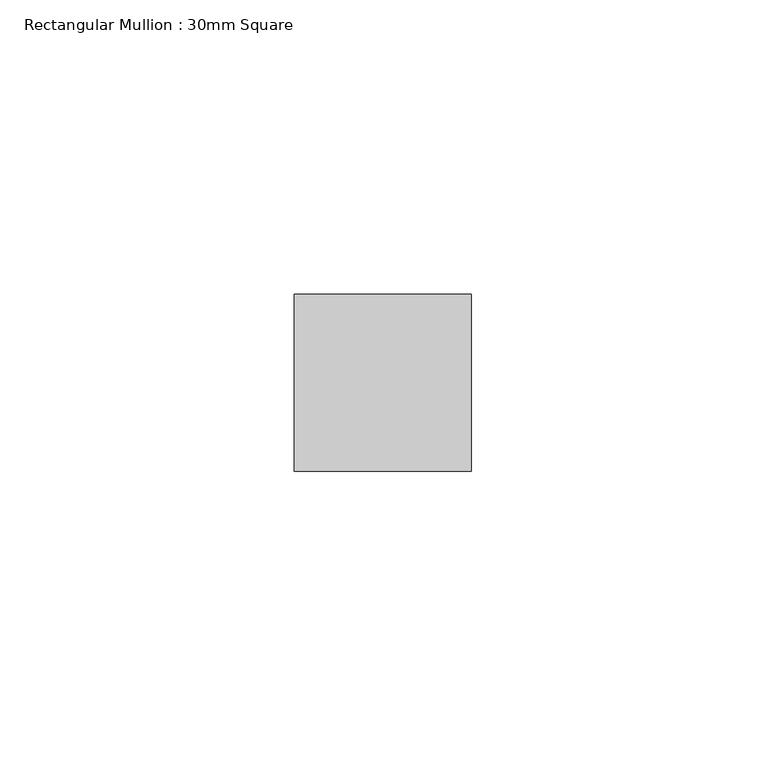
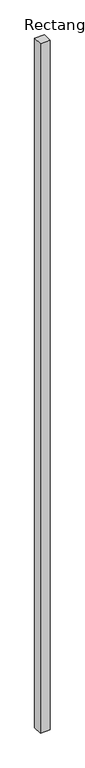
"""IFC4 building model written with IfcOpenShell, lengths in millimetres: member geometry, Rectangular Mullion : 30mm Square."""

from ifc_helpers import new_model, si_unit, frame, origin, place, context, project, spatial, polyline, outline, extrude, source, transform, mapped, element, save


def rectangular_mullion_30mm_square_b3fc8657(model_context):
    return source(origin(), model_context, "Body", "SweptSolid", [
        extrude(outline(polyline([(15.0, 15.0), (15.0, -15.0), (-15.0, -15.0), (-15.0, 15.0), (15.0, 15.0)])), frame((0.0, 0.0, -2256.188532), z_axis=(0.0, 0.0, 1.0), x_axis=(1.0, 0.0, 0.0)), (0.0, 0.0, 1.0), 2256.188532),
    ])


if __name__ == "__main__":
    model = new_model("IFC4")
    model_context = context("Model", 3, world=origin())
    ifc_project = project(units=[si_unit("LENGTHUNIT", "METRE", prefix="MILLI")], contexts=[model_context])
    site = spatial("IfcSite", under=ifc_project)
    building = spatial("IfcBuilding", under=site)
    placement = place(None, origin())
    rectangular_mullion_30mm_square_shape = rectangular_mullion_30mm_square_b3fc8657(model_context)
    element("IfcMember", 1, ObjectType="Rectangular Mullion : 30mm Square", at=placement, inside=building, context=model_context, shape_type="MappedRepresentation", body=[
        mapped(rectangular_mullion_30mm_square_shape, transform((0.0, 0.0, 0.0), x_axis=(1.0, 0.0, 0.0), y_axis=(0.0, 1.0, 0.0), z_axis=(0.0, 0.0, 1.0))),
    ])
    save(model, "model.ifc")

# Revit data of these elements
# Type "Rectangular Mullion : 30mm Square"
#   built-in parameter 1007304 = 0.0984252 (stored number, unit not read)
#   built-in parameter 1007301 = 0.0492126 (stored number, unit not read)
#   built-in parameter 1007300 = 0.0492126 (stored number, unit not read)
# Element 1 (IfcMember, "Rectangular Mullion : 30mm Square")
#   Materials on its faces: "Aluminum"
# Materials
#   "Aluminum": class "Metal", colour RGB 244 244 244, transparency 0, Description = "Aluminum 6061", Cost = 0
